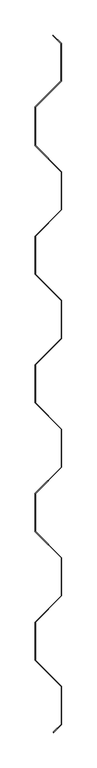
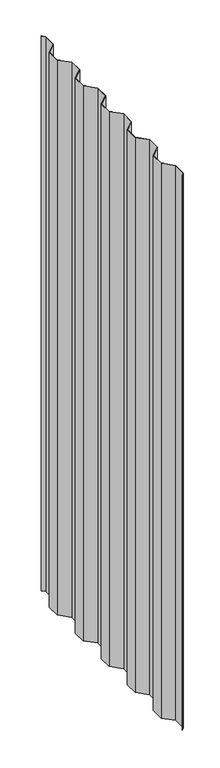
"""IFC4 building model written with IfcOpenShell, lengths in millimetres: proxy geometry, MBCI 7.2-V Panel5 : MBCI 7.2-V Panel-1."""

from ifc_helpers import new_model, si_unit, frame, origin, place, context, project, spatial, polyline, outline, extrude, source, transform, mapped, element, save


def generic_models_fc78e95f(model_context):
    return source(origin(), model_context, "Body", "SweptSolid", [
        extrude(outline(polyline([(587365.8648989, -535033.5731976), (587365.8648989, -535087.6849068), (587354.4642648, -535099.0855409), (587354.4223399, -535098.2855668), (587365.2695864, -535087.4383203), (587365.2695864, -535033.8197841), (587327.7791864, -534996.3293841), (587327.7791864, -534942.0487203), (587365.2695864, -534904.5583203), (587365.2695864, -534850.9397841), (587327.7791864, -534813.4493841), (587327.7791864, -534759.1687203), (587365.2695864, -534721.6783203), (587365.2695864, -534668.0597841), (587327.7791864, -534630.5693841), (587327.7791864, -534576.2887203), (587365.2695864, -534538.7983203), (587365.2695864, -534485.1797841), (587327.7791864, -534447.6893841), (587327.7791864, -534393.4087203), (587365.2695864, -534355.9183203), (587365.2695864, -534302.2997841), (587327.7791864, -534264.8093841), (587327.7791864, -534209.6651203), (587364.6599864, -534172.7843203), (587364.6599864, -534119.6961933), (587353.5295525, -534108.5657594), (587353.5845762, -534107.7788841), (587365.2552989, -534119.4496068), (587365.2552989, -534173.0309068), (587328.3744989, -534209.9117068), (587328.3744989, -534264.5627976), (587365.8648989, -534302.0531976), (587365.8648989, -534356.1649068), (587328.3744989, -534393.6553068), (587328.3744989, -534447.4427976), (587365.8648989, -534484.9331976), (587365.8648989, -534539.0449068), (587328.3744989, -534576.5353068), (587328.3744989, -534630.3227976), (587365.8648989, -534667.8131976), (587365.8648989, -534721.9249068), (587328.3744989, -534759.4153068), (587328.3744989, -534813.2027976), (587365.8648989, -534850.6931976), (587365.8648989, -534904.8049068), (587328.3744989, -534942.2953068), (587328.3744989, -534996.0827976), (587365.8648989, -535033.5731976)])), frame((0.0, 0.0, 51.59375), z_axis=(0.0, 0.0, 1.0), x_axis=(1.0, 0.0, 0.0)), (0.0, 0.0, 1.0), 2386.80625),
    ])


if __name__ == "__main__":
    model = new_model("IFC4")
    model_context = context("Model", 3, world=origin())
    ifc_project = project(units=[si_unit("LENGTHUNIT", "METRE", prefix="MILLI")], contexts=[model_context])
    site = spatial("IfcSite", under=ifc_project)
    building = spatial("IfcBuilding", under=site)
    placement = place(None, origin())
    generic_models_shape = generic_models_fc78e95f(model_context)
    element("IfcBuildingElementProxy", 1, Name="MBCI 7.2-V Panel5 : MBCI 7.2-V Panel-1", ObjectType="MBCI 7.2-V Panel5 : MBCI 7.2-V Panel-1", at=placement, inside=building, context=model_context, shape_type="MappedRepresentation", body=[
        mapped(generic_models_shape, transform((0.0, 0.0, 0.0), x_axis=(1.0, 0.0, 0.0), y_axis=(0.0, 1.0, 0.0), z_axis=(0.0, 0.0, 1.0))),
    ])
    save(model, "model.ifc")

# Revit data of these elements
# Element 1 (IfcBuildingElementProxy, "MBCI 7.2-V Panel5 : MBCI 7.2-V Panel-1")
#   Materials on its faces: "MTL PANEL"
# Materials
#   "MTL PANEL": class "Generic", colour RGB 239 242 240, transparency 0, Cost = 0
